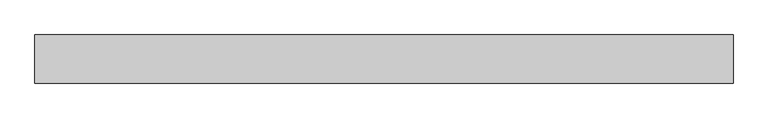
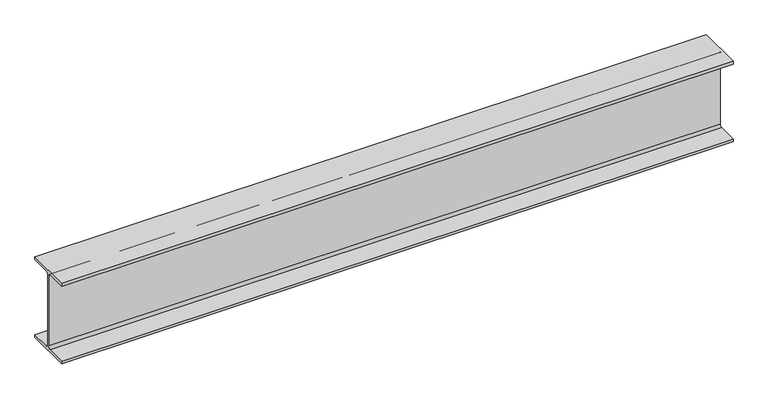
"""IFC4 building model written with IfcOpenShell, lengths in millimetres: beam geometry, Old_Steel Beam_H-KSD3502 : H_SB_ASB_H-194×150x6x9."""

from ifc_helpers import new_model, si_unit, point, frame, frame_2d, origin, place, context, project, spatial, polyline, circle_curve, trimmed, segment, composite_curve, outline, extrude, source, transform, mapped, element, save


def beam_260efa87(model_context):
    return source(origin(), model_context, "Body", "SweptSolid", [
        extrude(outline(composite_curve([segment(polyline([(-82.5, -141.5), (-11.9, -141.5)]), True, "CONTINUOUS"), segment(trimmed(circle_curve(frame_2d((-11.9, -132.6)), 8.9), [point((-11.9, -141.5))], [point((-3.0, -132.6))], True, "CARTESIAN"), True, "CONTINUOUS"), segment(polyline([(-3.0, -132.6), (-3.0, 132.6)]), True, "CONTINUOUS"), segment(trimmed(circle_curve(frame_2d((-11.9, 132.6)), 8.9), [point((-3.0, 132.6))], [point((-11.9, 141.5))], True, "CARTESIAN"), True, "CONTINUOUS"), segment(polyline([(-11.9, 141.5), (-82.5, 141.5), (-82.5, 151.7), (82.5, 151.7), (82.5, 141.5), (11.9, 141.5)]), True, "CONTINUOUS"), segment(trimmed(circle_curve(frame_2d((11.9, 132.6)), 8.9), [point((11.9, 141.5))], [point((3.0, 132.6))], True, "CARTESIAN"), True, "CONTINUOUS"), segment(polyline([(3.0, 132.6), (3.0, -132.6)]), True, "CONTINUOUS"), segment(trimmed(circle_curve(frame_2d((11.9, -132.6)), 8.9), [point((3.0, -132.6))], [point((11.9, -141.5))], True, "CARTESIAN"), True, "CONTINUOUS"), segment(polyline([(11.9, -141.5), (82.5, -141.5), (82.5, -151.7), (-82.5, -151.7), (-82.5, -141.5)]), True, "CONTINUOUS")], self_intersect=False)), frame((-1068.0314701, 0.0, 0.0), z_axis=(1.0, 0.0, 0.0), x_axis=(0.0, 1.0, 0.0)), (0.0, 0.0, 1.0), 2394.2341721),
    ])


if __name__ == "__main__":
    model = new_model("IFC4")
    model_context = context("Model", 3, world=origin())
    ifc_project = project(units=[si_unit("LENGTHUNIT", "METRE", prefix="MILLI")], contexts=[model_context])
    site = spatial("IfcSite", under=ifc_project)
    building = spatial("IfcBuilding", under=site)
    placement = place(None, origin())
    beam_shape = beam_260efa87(model_context)
    element("IfcBeam", 1, ObjectType="Old_Steel Beam_H-KSD3502 : H_SB_ASB_H-194×150x6x9", at=placement, inside=building, context=model_context, shape_type="MappedRepresentation", body=[
        mapped(beam_shape, transform((0.0, 0.0, 0.0), x_axis=(1.0, 0.0, 0.0), y_axis=(0.0, 1.0, 0.0), z_axis=(0.0, 0.0, 1.0))),
    ])
    save(model, "model.ifc")

# Revit data of these elements
# Type "Old_Steel Beam_H-KSD3502 : H_SB_ASB_H-194×150x6x9"
#   Width = 15.0 cm
#   Web Thickness = 0.6 cm
#   Web Fillet = 1.3 cm
#   Warping Constant = 43316.0 cm⁶
#   Torsional Moment of Inertia = 8.622 cm⁴
#   Torsional Modulus = 1.0 cm³
#   Section Area = 39.01 cm²
#   Plastic Modulus weak axis = 104.0 cm³
#   Plastic Modulus strong axis = 309.0 cm³
#   Perimeter = 0.95 m²/m
#   Nominal Weight = 30.60 kgf/m
#   Moment of Inertia weak axis = 507.00 cm⁴
#   Moment of Inertia strong axis = 2690.00 cm⁴
#   Height = 19.4 cm
#   Flange Thickness = 0.9 cm
#   Elastic Modulus weak axis = 67.6 cm³
#   Elastic Modulus strong axis = 277.0 cm³
#   Centroid Vertical = 9.7 cm
#   Centroid Horizontal = 7.5 cm
#   Length [instance default] = 1.5240 m
#   Structural Material [instance default] = Steel, 45-345
#   Assembly Code = ""
# Element 1 (IfcBeam, "Old_Steel Beam_H-KSD3502 : H_SB_ASB_H-194×150x6x9")
#   Structural Material = none
# Materials
#   "Steel, 45-345": class "Metal", colour RGB 189 187 185, transparency 0, Description = "Steel 345 MPa", Cost = 0
